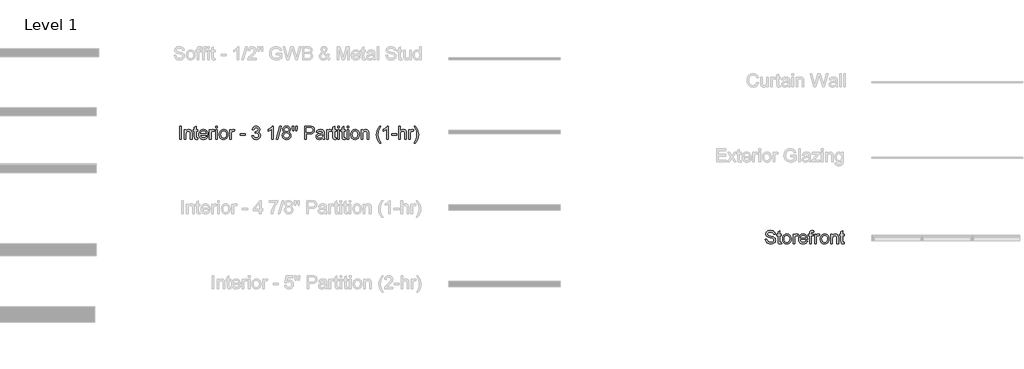
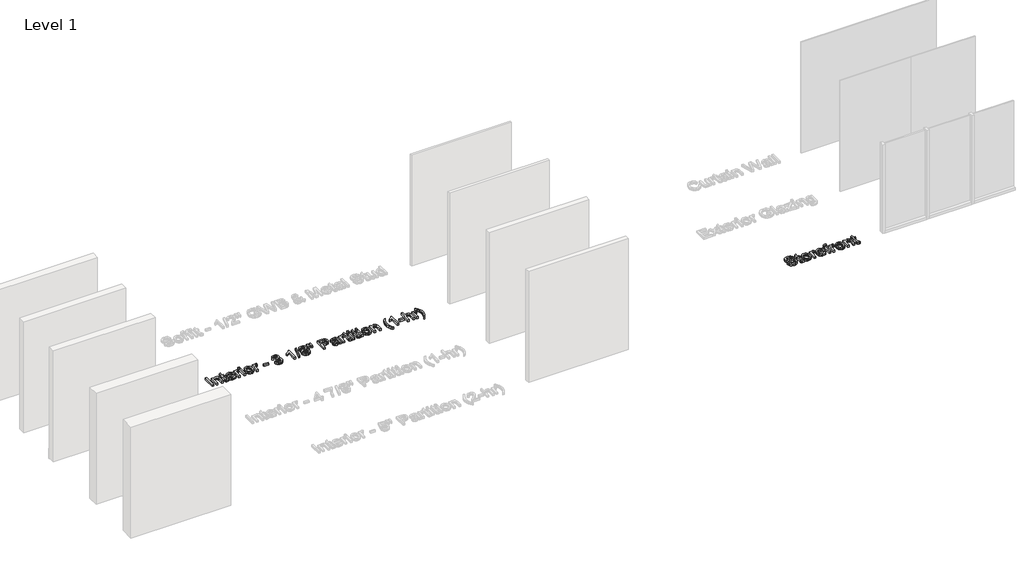
# One storey, part 36 of 42: 2 proxies.
"""IFC4 building model written with IfcOpenShell, lengths in millimetres."""

from ifc_helpers import new_model, si_unit, origin, origin_with_axes, place, context, project, spatial, polyline, outline, extrude, element, save

model = new_model("IFC4")

# Units and contexts
model_context = context("Model", 3, world=origin())
ifc_project = project(units=[si_unit("LENGTHUNIT", "METRE", prefix="MILLI")], contexts=[model_context])

# Site, building, storey
site = spatial("IfcSite", under=ifc_project)
building = spatial("IfcBuilding", under=site)
storey = spatial("IfcBuildingStorey", under=building, Name="Level 1", Elevation=0.0)

# Proxies
placement = place(None, origin())
element("IfcBuildingElementProxy", 1, Name="8\" Arial", ObjectType="8\" Arial", at=placement, inside=storey, context=model_context, shape_type="SweptSolid", body=[
    extrude(outline(polyline([(5241.2577476, 15464.2109771), (5241.2577476, 15768.7780711), (5279.3286344, 15768.7780711), (5279.3286344, 15464.2109771), (5241.2577476, 15464.2109771)])), origin_with_axes(), (0.0, 0.0, 1.0), 50.8),
    extrude(outline(polyline([(5350.711547, 15464.2109771), (5350.711547, 15687.8774368), (5388.7824338, 15687.8774368), (5388.7824338, 15656.6474125), (5402.0087209, 15672.3925497), (5417.8932779, 15683.6390763), (5436.4361048, 15690.3869923), (5457.6372016, 15692.6362976), (5476.4031002, 15690.8238408), (5493.5889082, 15685.3864705), (5507.9212586, 15677.0026962), (5518.1267844, 15666.3510272), (5529.5406147, 15638.3555411), (5531.5482591, 15601.5487268), (5531.5482591, 15464.2109771), (5493.4773724, 15464.2109771), (5493.4773724, 15596.4180799), (5489.0902975, 15630.1018918), (5483.020891, 15640.1308193), (5473.5868212, 15647.9104414), (5461.4944814, 15652.9016685), (5447.4502651, 15654.5654109), (5425.1523996, 15650.8289615), (5406.1448402, 15639.6196135), (5398.5487874, 15630.4690305), (5393.1230354, 15617.9630788), (5388.7824338, 15582.8850694), (5388.7824338, 15464.2109771), (5350.711547, 15464.2109771)])), origin_with_axes(), (0.0, 0.0, 1.0), 50.8),
    extrude(outline(polyline([(5664.7963628, 15495.9615018), (5669.5552236, 15463.0956191), (5641.0764158, 15459.4521162), (5622.8031337, 15461.0322067), (5609.1771767, 15465.7724783), (5599.5479192, 15473.0780732), (5593.2647357, 15482.354134), (5589.8071259, 15498.2851643), (5588.6545893, 15525.5556676), (5588.6545893, 15649.80655), (5560.1014242, 15649.80655), (5560.1014242, 15687.8774368), (5588.6545893, 15687.8774368), (5588.6545893, 15742.2325505), (5626.725476, 15764.6140679), (5626.725476, 15687.8774368), (5664.7963628, 15687.8774368), (5664.7963628, 15649.80655), (5626.725476, 15649.80655), (5626.725476, 15526.6710256), (5628.7331204, 15507.0407247), (5635.2393755, 15500.0883264), (5648.214707, 15497.523003), (5664.7963628, 15495.9615018)])), origin_with_axes(), (0.0, 0.0, 1.0), 50.8),
    extrude(outline(polyline([(5859.4635142, 15530.8350289), (5896.790829, 15526.076168), (5883.3414703, 15497.9505569), (5861.8801232, 15476.9260584), (5832.8901096, 15463.8206018), (5796.8547512, 15459.4521162), (5773.232398, 15461.3366065), (5752.1846629, 15466.9900774), (5733.7115459, 15476.412529), (5717.8130469, 15489.6039611), (5705.0282557, 15506.1972352), (5695.896262, 15525.8252125), (5690.4170658, 15548.4878931), (5688.590667, 15574.1852769), (5690.4356551, 15600.7540342), (5695.9706192, 15624.1719051), (5705.1955594, 15644.4388896), (5718.1104757, 15661.5549877), (5733.9671487, 15675.1530608), (5752.0173592, 15684.8659701), (5772.2611071, 15690.6937157), (5794.6983924, 15692.6362976), (5816.4130187, 15690.6983631), (5836.0502907, 15684.8845594), (5853.6102083, 15675.1948867), (5869.0927717, 15661.6293449), (5881.7311722, 15644.5504254), (5890.7586011, 15624.3206195), (5896.1750584, 15600.9399272), (5897.9805442, 15574.4083485), (5897.7574726, 15564.1470548), (5726.6615538, 15564.1470548), (5733.2514607, 15535.6496576), (5748.5597494, 15514.6995163), (5770.6531326, 15501.8171313), (5797.5983232, 15497.523003), (5817.8606604, 15499.5120581), (5834.925638, 15505.4792234), (5848.7932559, 15515.796285), (5859.4635142, 15530.8350289)]), holes=[polyline([(5726.6615538, 15602.2179416), (5859.9096574, 15602.2179416), (5854.7604213, 15622.3315644), (5844.6664313, 15636.7196827), (5822.4708069, 15650.1039788), (5794.549678, 15654.5654109), (5768.8871491, 15651.0055599), (5747.667463, 15640.3260069), (5732.9168533, 15623.6792886), (5726.6615538, 15602.2179416)])]), origin_with_axes(), (0.0, 0.0, 1.0), 50.8),
    extrude(outline(polyline([(5936.0514309, 15464.2109771), (5936.0514309, 15687.8774368), (5969.3634569, 15687.8774368), (5969.3634569, 15654.7884825), (5981.6695736, 15673.9726402), (5993.0090467, 15685.2749347), (6004.3856984, 15690.7959569), (6016.8033509, 15692.6362976), (6035.7644371, 15689.6991882), (6055.0229521, 15680.8878599), (6042.3078707, 15646.7579048), (6028.9235746, 15652.6135343), (6015.5392785, 15654.5654109), (6004.1719214, 15652.6878915), (5994.0128689, 15647.0553336), (5985.8056929, 15638.0952909), (5980.2939654, 15626.2353174), (5975.6652296, 15604.969158), (5974.1223177, 15581.7697114), (5974.1223177, 15464.2109771), (5936.0514309, 15464.2109771)])), origin_with_axes(), (0.0, 0.0, 1.0), 50.8),
    extrude(outline(polyline([(6078.8172563, 15730.7071844), (6078.8172563, 15768.7780711), (6116.888143, 15768.7780711), (6116.888143, 15730.7071844), (6078.8172563, 15730.7071844)])), origin_with_axes(), (0.0, 0.0, 1.0), 50.8),
    extrude(outline(polyline([(6078.8172563, 15464.2109771), (6078.8172563, 15687.8774368), (6116.888143, 15687.8774368), (6116.888143, 15464.2109771), (6078.8172563, 15464.2109771)])), origin_with_axes(), (0.0, 0.0, 1.0), 50.8),
    extrude(outline(polyline([(6164.4767515, 15576.0442069), (6166.5355165, 15605.0109839), (6172.7118115, 15629.9717667), (6183.0056364, 15650.9265553), (6197.4169914, 15667.8753498), (6211.9259402, 15678.7082645), (6227.9406223, 15686.4460607), (6245.4610377, 15691.0887384), (6264.4871864, 15692.6362976), (6285.490772, 15690.7518073), (6304.4820658, 15685.0983364), (6321.4610678, 15675.6758849), (6336.4277781, 15662.4844527), (6348.643272, 15645.9701832), (6357.3686248, 15626.5792194), (6362.6038364, 15604.3115615), (6364.348907, 15579.1672093), (6361.2630831, 15540.7059473), (6352.0056117, 15511.4277995), (6336.8460374, 15489.5017199), (6316.0539051, 15473.0966625), (6291.3580198, 15462.8632528), (6264.4871864, 15459.4521162), (6243.1768774, 15461.3296355), (6224.0089853, 15466.9621935), (6206.98351, 15476.3497901), (6192.1004516, 15489.4924253), (6180.0150828, 15506.1670276), (6171.3826765, 15526.1505252), (6166.2032327, 15549.4429184), (6164.4767515, 15576.0442069)]), holes=[polyline([(6202.5476383, 15576.1185641), (6206.9533024, 15541.6632962), (6220.1702948, 15517.1161254), (6240.060846, 15502.4212836), (6264.4871864, 15497.523003), (6288.8019911, 15502.4491675), (6308.6553637, 15517.2276612), (6321.8723561, 15542.1001448), (6326.2780202, 15577.3082793), (6321.8444721, 15610.759725), (6308.5438279, 15634.9722885), (6288.6625713, 15649.6671303), (6264.4871864, 15654.5654109), (6240.060846, 15649.6857196), (6220.1702948, 15635.0466457), (6206.9533024, 15610.5552427), (6202.5476383, 15576.1185641)])]), origin_with_axes(), (0.0, 0.0, 1.0), 50.8),
    extrude(outline(polyline([(6407.1786546, 15464.2109771), (6407.1786546, 15687.8774368), (6440.4906805, 15687.8774368), (6440.4906805, 15654.7884825), (6452.7967972, 15673.9726402), (6464.1362703, 15685.2749347), (6475.512922, 15690.7959569), (6487.9305745, 15692.6362976), (6506.8916607, 15689.6991882), (6526.1501757, 15680.8878599), (6513.4350944, 15646.7579048), (6500.0507983, 15652.6135343), (6486.6665021, 15654.5654109), (6475.2991451, 15652.6878915), (6465.1400925, 15647.0553336), (6456.9329165, 15638.0952909), (6451.421189, 15626.2353174), (6446.7924533, 15604.969158), (6445.2495413, 15581.7697114), (6445.2495413, 15464.2109771), (6407.1786546, 15464.2109771)])), origin_with_axes(), (0.0, 0.0, 1.0), 50.8),
    extrude(outline(polyline([(6649.8805577, 15554.6293331), (6649.8805577, 15592.7002199), (6768.8520788, 15592.7002199), (6768.8520788, 15554.6293331), (6649.8805577, 15554.6293331)])), origin_with_axes(), (0.0, 0.0, 1.0), 50.8),
    extrude(outline(polyline([(6921.1356258, 15545.1116114), (6959.2065126, 15549.8704723), (6967.7297067, 15525.9460429), (6980.2124218, 15509.7919411), (6997.2681047, 15500.5902375), (7019.5102023, 15497.523003), (7045.6095798, 15501.7427741), (7065.7603812, 15514.4020875), (7078.6427662, 15533.2888165), (7082.9368945, 15556.1908343), (7078.6799448, 15577.9310209), (7065.9090956, 15595.5629721), (7046.5762234, 15607.2463473), (7022.6332048, 15611.1408056), (6995.9389697, 15606.9768024), (7000.1773302, 15645.0476892), (7006.2746206, 15644.601546), (7029.0836919, 15647.3341731), (7049.4761542, 15655.5320545), (7063.8642726, 15669.3996724), (7068.660312, 15689.1415092), (7065.1841129, 15705.5837452), (7054.7555155, 15718.9215681), (7038.8430745, 15727.7607803), (7018.9153447, 15730.7071844), (6998.9504364, 15727.7328963), (6982.6290308, 15718.8100323), (6970.7132894, 15703.9385921), (6963.9653734, 15683.1185759), (6925.8944867, 15687.8774368), (6937.1038347, 15722.0631598), (6957.0501538, 15747.5862689), (6984.3392464, 15763.4801206), (7017.5769151, 15768.7780711), (7041.5106391, 15766.1662745), (7063.4924866, 15758.3308844), (7082.0260188, 15745.9689998), (7095.6147973, 15729.7777194), (7103.9520984, 15711.1233566), (7106.7311988, 15691.3722252), (7104.0915181, 15672.968818), (7096.1724763, 15656.2756265), (7083.0856089, 15642.0548118), (7064.942452, 15631.0685354), (7088.7739348, 15621.4392779), (7106.43377, 15605.0435152), (7117.3642785, 15582.7735336), (7121.0077813, 15555.5216195), (7119.1860299, 15536.2073366), (7113.7207756, 15518.4173764), (7104.6120185, 15502.1517387), (7091.8597586, 15487.4104237), (7076.323751, 15475.1786642), (7058.8637508, 15466.4416931), (7039.4797581, 15461.1995104), (7018.1717727, 15459.4521162), (6998.9132578, 15460.9439076), (6981.3649584, 15465.4192816), (6965.5268746, 15472.8782383), (6951.3990065, 15483.3207776), (6939.552975, 15496.1334528), (6930.560401, 15510.7028168), (6924.4212846, 15527.0288697), (6921.1356258, 15545.1116114)])), origin_with_axes(), (0.0, 0.0, 1.0), 50.8),
    extrude(outline(polyline([(7416.0571537, 15464.2109771), (7377.9862669, 15464.2109771), (7377.9862669, 15701.5591617), (7341.9230246, 15675.8687489), (7301.8444934, 15656.6474125), (7301.8444934, 15692.6362976), (7331.7453827, 15708.9019353), (7357.6495725, 15728.2533967), (7378.0699188, 15748.831752), (7391.5192774, 15768.7780711), (7416.0571537, 15768.7780711), (7416.0571537, 15464.2109771)])), origin_with_axes(), (0.0, 0.0, 1.0), 50.8),
    extrude(outline(polyline([(7487.4400664, 15464.2109771), (7573.0995616, 15768.7780711), (7607.4525883, 15768.7780711), (7521.7930931, 15464.2109771), (7487.4400664, 15464.2109771)])), origin_with_axes(), (0.0, 0.0, 1.0), 50.8),
    extrude(outline(polyline([(7680.9175026, 15631.9608218), (7660.5343349, 15641.9990439), (7646.2298684, 15655.6064117), (7637.7810315, 15672.5040855), (7634.9647525, 15692.413226), (7636.4983698, 15707.939939), (7641.0992216, 15722.1746956), (7648.7673079, 15735.1174958), (7659.5026288, 15746.7683397), (7672.7893311, 15756.3975972), (7688.1115617, 15763.2756383), (7724.8626082, 15768.7780711), (7761.8367262, 15763.1455132), (7777.3262606, 15756.1048157), (7790.8174452, 15746.2478393), (7801.7479537, 15734.3692765), (7809.5554598, 15721.2638199), (7814.2399634, 15706.9314694), (7815.8014646, 15691.3722252), (7813.0223643, 15672.1044156), (7804.6850631, 15655.4948759), (7790.6966148, 15641.97116), (7770.9640726, 15631.9608218), (7794.3958855, 15619.8870714), (7811.4515684, 15602.1064058), (7821.8522819, 15579.4739328), (7825.3191863, 15552.8447603), (7823.5996761, 15533.8557902), (7818.4411453, 15516.4469106), (7809.8435939, 15500.6181215), (7797.8070221, 15486.3694229), (7782.9634659, 15474.5931012), (7765.9449616, 15466.1814429), (7746.7515091, 15461.1344479), (7725.3831086, 15459.4521162), (7704.014708, 15461.1414189), (7684.8212556, 15466.2093268), (7667.8027513, 15474.6558401), (7652.9591951, 15486.4809587), (7640.9226232, 15500.8295747), (7632.3250719, 15516.8465805), (7627.1665411, 15534.531976), (7625.4470309, 15553.8857611), (7629.0533551, 15581.5466398), (7639.8723278, 15604.2999432), (7657.34627, 15621.3649207), (7680.9175026, 15631.9608218)]), holes=[polyline([(7663.5179176, 15555.2241907), (7665.1073028, 15540.659474), (7669.8754583, 15526.5594898), (7678.6774919, 15514.2626678), (7692.3685115, 15505.1074374), (7708.7642742, 15499.4191116), (7725.6805374, 15497.523003), (7751.5940218, 15501.5104079), (7771.0384298, 15513.4726225), (7783.1958321, 15531.5878955), (7787.2482996, 15554.0344755), (7783.065707, 15576.8621361), (7770.5179294, 15595.3770791), (7750.6273782, 15607.6460172), (7724.416465, 15611.7356633), (7698.8654719, 15607.7017851), (7679.6162516, 15595.6001507), (7667.5425011, 15577.4384044), (7663.5179176, 15555.2241907)]), polyline([(7673.0356393, 15691.297868), (7676.4095973, 15674.6790336), (7686.5314712, 15661.4062733), (7703.1038323, 15652.7064808), (7725.8292518, 15649.80655), (7748.0248762, 15652.6878915), (7764.3462818, 15661.3319161), (7774.3845039, 15674.1585332), (7777.7305779, 15689.5876524), (7774.2729681, 15705.6023345), (7763.9001386, 15718.8472109), (7747.3556614, 15727.742191), (7725.3831086, 15730.7071844), (7703.271136, 15727.8072535), (7686.7545428, 15719.1074611), (7676.4653652, 15706.3552011), (7673.0356393, 15691.297868)])]), origin_with_axes(), (0.0, 0.0, 1.0), 50.8),
    extrude(outline(polyline([(7867.9258623, 15659.3242717), (7858.6312122, 15718.1408175), (7858.6312122, 15768.7780711), (7896.702099, 15768.7780711), (7896.702099, 15718.1408175), (7888.3740925, 15659.3242717), (7867.9258623, 15659.3242717)])), origin_with_axes(), (0.0, 0.0, 1.0), 50.8),
    extrude(outline(polyline([(7943.8445643, 15659.3242717), (7934.7729858, 15718.1408175), (7934.7729858, 15768.7780711), (7972.8438725, 15768.7780711), (7972.8438725, 15718.1408175), (7963.9210084, 15659.3242717), (7943.8445643, 15659.3242717)])), origin_with_axes(), (0.0, 0.0, 1.0), 50.8),
    extrude(outline(polyline([(8144.1628629, 15464.2109771), (8144.1628629, 15768.7780711), (8257.0370936, 15768.7780711), (8302.5437004, 15765.8781403), (8322.8339216, 15760.4593593), (8339.5364078, 15751.6387364), (8352.9857665, 15739.0166015), (8363.516605, 15722.1932849), (8370.3202889, 15702.349207), (8372.5881835, 15680.6647883), (8371.0568899, 15661.9685996), (8366.4630091, 15644.7688497), (8358.8065411, 15629.0655383), (8348.0874859, 15614.8586657), (8333.3717311, 15603.082344), (8313.7251645, 15594.6706857), (8289.147786, 15589.6236907), (8259.6395956, 15587.941359), (8182.2337497, 15587.941359), (8182.2337497, 15464.2109771), (8144.1628629, 15464.2109771)]), holes=[polyline([(8182.2337497, 15626.0122458), (8261.8703116, 15626.0122458), (8295.6284808, 15629.5070342), (8317.935641, 15639.9913995), (8330.3718828, 15656.8147162), (8334.5172967, 15679.3263587), (8332.0728038, 15696.4285148), (8324.7393248, 15710.8538118), (8313.4277357, 15721.7099631), (8299.048912, 15728.1046823), (8260.9780252, 15730.7071844), (8182.2337497, 15730.7071844), (8182.2337497, 15626.0122458)])]), origin_with_axes(), (0.0, 0.0, 1.0), 50.8),
    extrude(outline(polyline([(8562.9426173, 15492.7641421), (8544.7529871, 15477.1677193), (8526.0242671, 15466.9621935), (8506.3289036, 15461.3296355), (8485.2393426, 15459.4521162), (8453.4237553, 15463.9693162), (8429.9547638, 15477.520916), (8415.4829936, 15498.0992713), (8410.6590702, 15523.6967376), (8412.4808217, 15539.4790535), (8417.9460759, 15553.8114039), (8426.3763235, 15566.080342), (8437.0930551, 15575.6724209), (8463.7501115, 15588.1644306), (8496.6903515, 15593.8899351), (8535.616346, 15599.9128683), (8562.7195457, 15606.9768024), (8562.9426173, 15615.4535233), (8560.321526, 15632.4441436), (8552.458252, 15643.5605451), (8534.872774, 15651.8141944), (8510.3720764, 15654.5654109), (8487.6931302, 15652.7343648), (8471.8550464, 15647.2412266), (8461.054663, 15637.082174), (8453.4888179, 15621.2533849), (8415.4179311, 15626.0122458), (8422.0264273, 15646.832262), (8431.888051, 15663.1908461), (8445.9229727, 15675.7014452), (8465.0513626, 15684.9775059), (8488.4459968, 15690.7215997), (8515.2796516, 15692.6362976), (8541.0165377, 15690.9446713), (8561.4182947, 15685.8697923), (8576.8009406, 15678.2388846), (8587.4804935, 15668.879172), (8594.5630169, 15657.3073326), (8599.154574, 15643.0400447), (8601.013504, 15609.7280188), (8601.013504, 15562.362482), (8602.9467913, 15496.221752), (8610.5312257, 15464.2109771), (8572.460339, 15464.2109771), (8566.3630485, 15477.4465588), (8562.9426173, 15492.7641421)]), holes=[polyline([(8562.9426173, 15568.9059156), (8501.5235695, 15557.2318351), (8468.7692226, 15551.0601875), (8453.9349611, 15541.0219654), (8448.729957, 15526.3735968), (8451.5648253, 15515.052713), (8460.0694301, 15505.7766523), (8474.0578785, 15499.5864153), (8493.3442774, 15497.523003), (8513.7925076, 15499.8001922), (8531.8613074, 15506.6317601), (8546.5096759, 15516.6978661), (8556.6966124, 15528.6786701), (8561.2138124, 15541.0219654), (8562.7195457, 15558.1241215), (8562.9426173, 15568.9059156)])]), origin_with_axes(), (0.0, 0.0, 1.0), 50.8),
    extrude(outline(polyline([(8653.3609733, 15464.2109771), (8653.3609733, 15687.8774368), (8686.6729992, 15687.8774368), (8686.6729992, 15654.7884825), (8698.979116, 15673.9726402), (8710.3185891, 15685.2749347), (8721.6952408, 15690.7959569), (8734.1128933, 15692.6362976), (8753.0739795, 15689.6991882), (8772.3324945, 15680.8878599), (8759.6174131, 15646.7579048), (8746.233117, 15652.6135343), (8732.8488209, 15654.5654109), (8721.4814638, 15652.6878915), (8711.3224113, 15647.0553336), (8703.1152353, 15638.0952909), (8697.6035078, 15626.2353174), (8692.974772, 15604.969158), (8691.4318601, 15581.7697114), (8691.4318601, 15464.2109771), (8653.3609733, 15464.2109771)])), origin_with_axes(), (0.0, 0.0, 1.0), 50.8),
    extrude(outline(polyline([(8877.027433, 15495.9615018), (8881.7862939, 15463.0956191), (8853.307486, 15459.4521162), (8835.0342039, 15461.0322067), (8821.4082469, 15465.7724783), (8811.7789894, 15473.0780732), (8805.495806, 15482.354134), (8802.0381961, 15498.2851643), (8800.8856595, 15525.5556676), (8800.8856595, 15649.80655), (8772.3324945, 15649.80655), (8772.3324945, 15687.8774368), (8800.8856595, 15687.8774368), (8800.8856595, 15742.2325505), (8838.9565463, 15764.6140679), (8838.9565463, 15687.8774368), (8877.027433, 15687.8774368), (8877.027433, 15649.80655), (8838.9565463, 15649.80655), (8838.9565463, 15526.6710256), (8840.9641907, 15507.0407247), (8847.4704458, 15500.0883264), (8860.4457773, 15497.523003), (8877.027433, 15495.9615018)])), origin_with_axes(), (0.0, 0.0, 1.0), 50.8),
    extrude(outline(polyline([(8915.0983198, 15730.7071844), (8915.0983198, 15768.7780711), (8953.1692066, 15768.7780711), (8953.1692066, 15730.7071844), (8915.0983198, 15730.7071844)])), origin_with_axes(), (0.0, 0.0, 1.0), 50.8),
    extrude(outline(polyline([(8915.0983198, 15464.2109771), (8915.0983198, 15687.8774368), (8953.1692066, 15687.8774368), (8953.1692066, 15464.2109771), (8915.0983198, 15464.2109771)])), origin_with_axes(), (0.0, 0.0, 1.0), 50.8),
    extrude(outline(polyline([(9091.1761711, 15495.9615018), (9095.9350319, 15463.0956191), (9067.456224, 15459.4521162), (9049.182942, 15461.0322067), (9035.5569849, 15465.7724783), (9025.9277274, 15473.0780732), (9019.644544, 15482.354134), (9016.1869342, 15498.2851643), (9015.0343975, 15525.5556676), (9015.0343975, 15649.80655), (8986.4812325, 15649.80655), (8986.4812325, 15687.8774368), (9015.0343975, 15687.8774368), (9015.0343975, 15742.2325505), (9053.1052843, 15764.6140679), (9053.1052843, 15687.8774368), (9091.1761711, 15687.8774368), (9091.1761711, 15649.80655), (9053.1052843, 15649.80655), (9053.1052843, 15526.6710256), (9055.1129287, 15507.0407247), (9061.6191838, 15500.0883264), (9074.5945153, 15497.523003), (9091.1761711, 15495.9615018)])), origin_with_axes(), (0.0, 0.0, 1.0), 50.8),
    extrude(outline(polyline([(9129.2470578, 15464.2109771), (9129.2470578, 15687.8774368), (9167.3179446, 15687.8774368), (9167.3179446, 15464.2109771), (9129.2470578, 15464.2109771)])), origin_with_axes(), (0.0, 0.0, 1.0), 50.8),
    extrude(outline(polyline([(9129.2470578, 15730.7071844), (9129.2470578, 15768.7780711), (9167.3179446, 15768.7780711), (9167.3179446, 15730.7071844), (9129.2470578, 15730.7071844)])), origin_with_axes(), (0.0, 0.0, 1.0), 50.8),
    extrude(outline(polyline([(9214.906553, 15576.0442069), (9216.965318, 15605.0109839), (9223.141613, 15629.9717667), (9233.435438, 15650.9265553), (9247.8467929, 15667.8753498), (9262.3557417, 15678.7082645), (9278.3704238, 15686.4460607), (9295.8908392, 15691.0887384), (9314.916988, 15692.6362976), (9335.9205735, 15690.7518073), (9354.9118673, 15685.0983364), (9371.8908693, 15675.6758849), (9386.8575796, 15662.4844527), (9399.0730735, 15645.9701832), (9407.7984263, 15626.5792194), (9413.033638, 15604.3115615), (9414.7787085, 15579.1672093), (9411.6928847, 15540.7059473), (9402.4354132, 15511.4277995), (9387.2758389, 15489.5017199), (9366.4837066, 15473.0966625), (9341.7878214, 15462.8632528), (9314.916988, 15459.4521162), (9293.606679, 15461.3296355), (9274.4387868, 15466.9621935), (9257.4133115, 15476.3497901), (9242.5302531, 15489.4924253), (9230.4448843, 15506.1670276), (9221.812478, 15526.1505252), (9216.6330343, 15549.4429184), (9214.906553, 15576.0442069)]), holes=[polyline([(9252.9774398, 15576.1185641), (9257.3831039, 15541.6632962), (9270.6000963, 15517.1161254), (9290.4906475, 15502.4212836), (9314.916988, 15497.523003), (9339.2317926, 15502.4491675), (9359.0851652, 15517.2276612), (9372.3021576, 15542.1001448), (9376.7078217, 15577.3082793), (9372.2742737, 15610.759725), (9358.9736294, 15634.9722885), (9339.0923728, 15649.6671303), (9314.916988, 15654.5654109), (9290.4906475, 15649.6857196), (9270.6000963, 15635.0466457), (9257.3831039, 15610.5552427), (9252.9774398, 15576.1185641)])]), origin_with_axes(), (0.0, 0.0, 1.0), 50.8),
    extrude(outline(polyline([(9457.6084561, 15464.2109771), (9457.6084561, 15687.8774368), (9495.6793429, 15687.8774368), (9495.6793429, 15656.6474125), (9508.9056299, 15672.3925497), (9524.7901869, 15683.6390763), (9543.3330139, 15690.3869923), (9564.5341107, 15692.6362976), (9583.3000092, 15690.8238408), (9600.4858173, 15685.3864705), (9614.8181677, 15677.0026962), (9625.0236935, 15666.3510272), (9636.4375238, 15638.3555411), (9638.4451682, 15601.5487268), (9638.4451682, 15464.2109771), (9600.3742815, 15464.2109771), (9600.3742815, 15596.4180799), (9595.9872066, 15630.1018918), (9589.9178001, 15640.1308193), (9580.4837303, 15647.9104414), (9568.3913905, 15652.9016685), (9554.3471742, 15654.5654109), (9532.0493087, 15650.8289615), (9513.0417492, 15639.6196135), (9505.4456964, 15630.4690305), (9500.0199445, 15617.9630788), (9495.6793429, 15582.8850694), (9495.6793429, 15464.2109771), (9457.6084561, 15464.2109771)])), origin_with_axes(), (0.0, 0.0, 1.0), 50.8),
    extrude(outline(polyline([(9885.9059321, 15378.5514819), (9856.4047128, 15419.9498533), (9831.8482472, 15467.8544799), (9815.2851808, 15519.941699), (9809.7641586, 15573.8878481), (9813.8909833, 15621.197617), (9826.2714572, 15666.462563), (9850.846512, 15717.7318528), (9885.9059321, 15768.7780711), (9914.4590972, 15768.7780711), (9878.8419981, 15708.4743814), (9857.4271243, 15650.0296216), (9850.2330651, 15611.9401456), (9847.8350454, 15573.6647765), (9851.9990486, 15524.8585689), (9864.4910583, 15476.0709506), (9885.3110745, 15427.3019216), (9914.4590972, 15378.5514819), (9885.9059321, 15378.5514819)])), origin_with_axes(), (0.0, 0.0, 1.0), 50.8),
    extrude(outline(polyline([(10085.7780876, 15464.2109771), (10047.7072009, 15464.2109771), (10047.7072009, 15701.5591617), (10011.6439585, 15675.8687489), (9971.5654273, 15656.6474125), (9971.5654273, 15692.6362976), (10001.4663167, 15708.9019353), (10027.3705065, 15728.2533967), (10047.7908527, 15748.831752), (10061.2402114, 15768.7780711), (10085.7780876, 15768.7780711), (10085.7780876, 15464.2109771)])), origin_with_axes(), (0.0, 0.0, 1.0), 50.8),
    extrude(outline(polyline([(10166.678722, 15554.6293331), (10166.678722, 15592.7002199), (10285.6502431, 15592.7002199), (10285.6502431, 15554.6293331), (10166.678722, 15554.6293331)])), origin_with_axes(), (0.0, 0.0, 1.0), 50.8),
    extrude(outline(polyline([(10328.4799907, 15464.2109771), (10328.4799907, 15768.7780711), (10366.5508775, 15768.7780711), (10366.5508775, 15656.7961269), (10380.5346785, 15672.4762016), (10396.2379898, 15683.6762549), (10413.6608114, 15690.3962869), (10432.8031433, 15692.6362976), (10455.7981076, 15690.1918046), (10475.5585337, 15682.8583257), (10491.1177779, 15671.2121292), (10501.5091967, 15655.8294833), (10507.3648263, 15634.693449), (10509.3167028, 15605.7870872), (10509.3167028, 15464.2109771), (10471.2458161, 15464.2109771), (10471.2458161, 15601.8461556), (10468.2157601, 15625.6776384), (10459.1255923, 15641.9990439), (10444.4772238, 15651.4238191), (10424.7725656, 15654.5654109), (10408.6835263, 15652.4462306), (10393.5797199, 15646.08869), (10381.0691209, 15636.1062358), (10372.7597037, 15623.112315), (10368.103084, 15605.8428551), (10366.5508775, 15583.0337838), (10366.5508775, 15464.2109771), (10328.4799907, 15464.2109771)])), origin_with_axes(), (0.0, 0.0, 1.0), 50.8),
    extrude(outline(polyline([(10561.6641721, 15464.2109771), (10561.6641721, 15687.8774368), (10594.976198, 15687.8774368), (10594.976198, 15654.7884825), (10607.2823147, 15673.9726402), (10618.6217878, 15685.2749347), (10629.9984395, 15690.7959569), (10642.4160921, 15692.6362976), (10661.3771782, 15689.6991882), (10680.6356932, 15680.8878599), (10667.9206119, 15646.7579048), (10654.5363158, 15652.6135343), (10641.1520197, 15654.5654109), (10629.7846626, 15652.6878915), (10619.6256101, 15647.0553336), (10611.418434, 15638.0952909), (10605.9067065, 15626.2353174), (10601.2779708, 15604.969158), (10599.7350589, 15581.7697114), (10599.7350589, 15464.2109771), (10561.6641721, 15464.2109771)])), origin_with_axes(), (0.0, 0.0, 1.0), 50.8),
    extrude(outline(polyline([(10713.9477191, 15378.5514819), (10685.3945541, 15378.5514819), (10714.5425767, 15427.3019216), (10735.3625929, 15476.0709506), (10747.8546027, 15524.8585689), (10752.0186059, 15573.6647765), (10749.6205862, 15611.661306), (10742.426527, 15649.3604068), (10733.3363592, 15679.2334122), (10721.2347248, 15707.8795238), (10685.3945541, 15768.7780711), (10713.9477191, 15768.7780711), (10749.0071393, 15717.7318528), (10773.5821941, 15666.462563), (10785.962668, 15621.197617), (10790.0894927, 15573.8878481), (10784.5405866, 15519.941699), (10767.8938682, 15467.8544799), (10743.3095188, 15419.9498533), (10713.9477191, 15378.5514819)])), origin_with_axes(), (0.0, 0.0, 1.0), 50.8),
])
element("IfcBuildingElementProxy", 2, Name="8\" Arial", ObjectType="8\" Arial", at=placement, inside=storey, context=model_context, shape_type="SweptSolid", body=[
    extrude(outline(polyline([(18840.5112863, 13143.7956167), (18878.582173, 13143.7956167), (18882.9506586, 13122.6688771), (18890.8511111, 13105.6875513), (18903.1758171, 13092.2103087), (18920.817063, 13081.5958183), (18942.3806512, 13074.7084826), (18966.4723842, 13072.412704), (18987.6827757, 13074.1508036), (19006.2534866, 13079.3651023), (19021.3015251, 13087.6187516), (19031.9438995, 13098.4749029), (19038.2735562, 13110.9390286), (19040.3834417, 13124.0166013), (19038.8033512, 13136.7595666), (19034.0630797, 13147.7737269), (19024.4338222, 13157.1706182), (19008.1867738, 13165.0617761), (18952.7534807, 13179.5986088), (18916.3649256, 13189.2185717), (18893.0818271, 13198.373802), (18874.1300356, 13211.1818298), (18860.6992662, 13226.7038955), (18852.6965725, 13244.6053916), (18850.0290079, 13264.5517106), (18853.3286087, 13286.8495762), (18863.2274111, 13307.6417085), (18879.4651648, 13325.264365), (18901.7816196, 13338.0538035), (18928.5688012, 13345.8334257), (18958.218735, 13348.426633), (18990.3410457, 13345.7125952), (19018.4480675, 13337.5704817), (19041.5359783, 13324.1675963), (19058.6009559, 13305.6712426), (19069.4013393, 13283.2339573), (19073.6954676, 13258.008277), (19035.6245809, 13258.008277), (19028.635004, 13280.7244018), (19014.0609927, 13297.1201646), (18991.2891, 13307.0468508), (18959.705879, 13310.3557463), (18927.379086, 13307.0840294), (18905.2020509, 13297.268879), (18892.3754337, 13282.8249927), (18888.0998947, 13265.6670687), (18891.1299506, 13251.0372894), (18900.2201184, 13239.2702624), (18921.7093494, 13228.7487185), (18962.3827382, 13218.004103), (19004.357378, 13207.7985772), (19029.750362, 13198.8943024), (19051.45337, 13185.0824524), (19066.594355, 13168.0360641), (19075.4893351, 13147.9410306), (19078.4543285, 13124.9832449), (19075.0431919, 13101.5142535), (19064.8097822, 13079.4394595), (19048.1723585, 13060.4411947), (19025.5491802, 13046.2017908), (18998.3437394, 13037.3068107), (18967.9595283, 13034.3418173), (18930.6600975, 13037.5391769), (18899.9598682, 13047.1312558), (18875.5056438, 13063.1552325), (18856.9442276, 13085.6482858), (18845.0284862, 13113.0489142), (18840.5112863, 13143.7956167)])), origin_with_axes(), (0.0, 0.0, 1.0), 50.8),
    extrude(outline(polyline([(19211.7024321, 13070.8512028), (19216.461293, 13037.9853201), (19187.9824851, 13034.3418173), (19169.7092031, 13035.9219078), (19156.083246, 13040.6621793), (19146.4539885, 13047.9677743), (19140.1708051, 13057.2438351), (19136.7131952, 13073.1748653), (19135.5606586, 13100.4453687), (19135.5606586, 13224.6962511), (19107.0074936, 13224.6962511), (19107.0074936, 13262.7671378), (19135.5606586, 13262.7671378), (19135.5606586, 13317.1222515), (19173.6315454, 13339.503769), (19173.6315454, 13262.7671378), (19211.7024321, 13262.7671378), (19211.7024321, 13224.6962511), (19173.6315454, 13224.6962511), (19173.6315454, 13101.5607267), (19175.6391898, 13081.9304257), (19182.1454449, 13074.9780275), (19195.1207764, 13072.412704), (19211.7024321, 13070.8512028)])), origin_with_axes(), (0.0, 0.0, 1.0), 50.8),
    extrude(outline(polyline([(19240.2555972, 13150.933908), (19242.3143622, 13179.900685), (19248.4906572, 13204.8614678), (19258.7844822, 13225.8162564), (19273.1958371, 13242.7650508), (19287.7047859, 13253.5979655), (19303.719468, 13261.3357617), (19321.2398834, 13265.9784394), (19340.2660322, 13267.5259987), (19361.2696177, 13265.6415084), (19380.2609115, 13259.9880375), (19397.2399135, 13250.5655859), (19412.2066238, 13237.3741538), (19424.4221177, 13220.8598842), (19433.1474705, 13201.4689205), (19438.3826821, 13179.2012626), (19440.1277527, 13154.0569104), (19437.0419289, 13115.5956483), (19427.7844574, 13086.3175006), (19412.6248831, 13064.391421), (19391.8327508, 13047.9863636), (19367.1368656, 13037.7529539), (19340.2660322, 13034.3418173), (19318.9557232, 13036.2193366), (19299.787831, 13041.8518945), (19282.7623557, 13051.2394911), (19267.8792973, 13064.3821264), (19255.7939285, 13081.0567286), (19247.1615222, 13101.0402263), (19241.9820785, 13124.3326194), (19240.2555972, 13150.933908)]), holes=[polyline([(19278.326484, 13151.0082652), (19282.7321481, 13116.5529973), (19295.9491405, 13092.0058264), (19315.8396917, 13077.3109846), (19340.2660322, 13072.412704), (19364.5808368, 13077.3388686), (19384.4342094, 13092.1173622), (19397.6512018, 13116.9898459), (19402.0568659, 13152.1979804), (19397.6233178, 13185.6494261), (19384.3226736, 13209.8619895), (19364.441417, 13224.5568313), (19340.2660322, 13229.4551119), (19315.8396917, 13224.5754206), (19295.9491405, 13209.9363467), (19282.7321481, 13185.4449438), (19278.326484, 13151.0082652)])]), origin_with_axes(), (0.0, 0.0, 1.0), 50.8),
    extrude(outline(polyline([(19482.9575003, 13039.1006781), (19482.9575003, 13262.7671378), (19516.2695262, 13262.7671378), (19516.2695262, 13229.6781835), (19528.5756429, 13248.8623413), (19539.915116, 13260.1646358), (19551.2917677, 13265.685658), (19563.7094203, 13267.5259987), (19582.6705064, 13264.5888892), (19601.9290214, 13255.777561), (19589.2139401, 13221.6476058), (19575.829644, 13227.5032354), (19562.4453479, 13229.4551119), (19551.0779908, 13227.5775926), (19540.9189382, 13221.9450346), (19532.7117622, 13212.984992), (19527.2000347, 13201.1250184), (19522.571299, 13179.858859), (19521.0283871, 13156.6594124), (19521.0283871, 13039.1006781), (19482.9575003, 13039.1006781)])), origin_with_axes(), (0.0, 0.0, 1.0), 50.8),
    extrude(outline(polyline([(19782.3195903, 13105.7247299), (19819.6469051, 13100.9658691), (19806.1975464, 13072.8402579), (19784.7361993, 13051.8157594), (19755.7461857, 13038.7103028), (19719.7108273, 13034.3418173), (19696.0884741, 13036.2263076), (19675.040739, 13041.8797785), (19656.567622, 13051.30223), (19640.669123, 13064.4936622), (19627.8843318, 13081.0869362), (19618.7523381, 13100.7149136), (19613.2731419, 13123.3775941), (19611.4467431, 13149.074978), (19613.2917312, 13175.6437352), (19618.8266953, 13199.0616061), (19628.0516355, 13219.3285906), (19640.9665518, 13236.4446888), (19656.8232248, 13250.0427619), (19674.8734353, 13259.7556712), (19695.1171832, 13265.5834168), (19717.5544685, 13267.5259987), (19739.2690948, 13265.5880641), (19758.9063668, 13259.7742605), (19776.4662844, 13250.0845878), (19791.9488478, 13236.519046), (19804.5872483, 13219.4401264), (19813.6146772, 13199.2103205), (19819.0311345, 13175.8296282), (19820.8366203, 13149.2980496), (19820.6135487, 13139.0367559), (19649.5176299, 13139.0367559), (19656.1075368, 13110.5393587), (19671.4158255, 13089.5892174), (19693.5092087, 13076.7068324), (19720.4543993, 13072.412704), (19740.7167365, 13074.4017592), (19757.7817141, 13080.3689245), (19771.649332, 13090.6859861), (19782.3195903, 13105.7247299)]), holes=[polyline([(19649.5176299, 13177.1076426), (19782.7657335, 13177.1076426), (19777.6164974, 13197.2212654), (19767.5225074, 13211.6093837), (19745.326883, 13224.9936799), (19717.4057541, 13229.4551119), (19691.7432252, 13225.8952609), (19670.5235391, 13215.215708), (19655.7729294, 13198.5689897), (19649.5176299, 13177.1076426)])]), origin_with_axes(), (0.0, 0.0, 1.0), 50.8),
    extrude(outline(polyline([(19868.4252287, 13039.1006781), (19868.4252287, 13224.6962511), (19835.1132028, 13224.6962511), (19835.1132028, 13262.7671378), (19868.4252287, 13262.7671378), (19868.4252287, 13285.2973696), (19872.4405176, 13317.0478943), (19880.0993092, 13329.7072078), (19891.9221042, 13339.7268406), (19908.4665813, 13346.2516849), (19930.2904197, 13348.426633), (19965.0152324, 13344.2626298), (19959.4384424, 13308.5711735), (19937.5030682, 13310.3557463), (19923.031298, 13308.7756558), (19913.522871, 13304.0353842), (19908.2528044, 13294.982395), (19906.4961155, 13280.4641516), (19906.4961155, 13262.7671378), (19949.3258631, 13262.7671378), (19949.3258631, 13224.6962511), (19906.4961155, 13224.6962511), (19906.4961155, 13039.1006781), (19868.4252287, 13039.1006781)])), origin_with_axes(), (0.0, 0.0, 1.0), 50.8),
    extrude(outline(polyline([(19982.637889, 13039.1006781), (19982.637889, 13262.7671378), (20015.9499149, 13262.7671378), (20015.9499149, 13229.6781835), (20028.2560316, 13248.8623413), (20039.5955047, 13260.1646358), (20050.9721565, 13265.685658), (20063.389809, 13267.5259987), (20082.3508951, 13264.5888892), (20101.6094101, 13255.777561), (20088.8943288, 13221.6476058), (20075.5100327, 13227.5032354), (20062.1257366, 13229.4551119), (20050.7583795, 13227.5775926), (20040.599327, 13221.9450346), (20032.3921509, 13212.984992), (20026.8804234, 13201.1250184), (20022.2516877, 13179.858859), (20020.7087758, 13156.6594124), (20020.7087758, 13039.1006781), (19982.637889, 13039.1006781)])), origin_with_axes(), (0.0, 0.0, 1.0), 50.8),
    extrude(outline(polyline([(20115.8859927, 13150.933908), (20117.9447577, 13179.900685), (20124.1210526, 13204.8614678), (20134.4148776, 13225.8162564), (20148.8262326, 13242.7650508), (20163.3351814, 13253.5979655), (20179.3498635, 13261.3357617), (20196.8702789, 13265.9784394), (20215.8964276, 13267.5259987), (20236.9000131, 13265.6415084), (20255.8913069, 13259.9880375), (20272.870309, 13250.5655859), (20287.8370193, 13237.3741538), (20300.0525132, 13220.8598842), (20308.7778659, 13201.4689205), (20314.0130776, 13179.2012626), (20315.7581481, 13154.0569104), (20312.6723243, 13115.5956483), (20303.4148528, 13086.3175006), (20288.2552785, 13064.391421), (20267.4631463, 13047.9863636), (20242.767261, 13037.7529539), (20215.8964276, 13034.3418173), (20194.5861186, 13036.2193366), (20175.4182265, 13041.8518945), (20158.3927512, 13051.2394911), (20143.5096927, 13064.3821264), (20131.4243239, 13081.0567286), (20122.7919177, 13101.0402263), (20117.6124739, 13124.3326194), (20115.8859927, 13150.933908)]), holes=[polyline([(20153.9568794, 13151.0082652), (20158.3625436, 13116.5529973), (20171.579536, 13092.0058264), (20191.4700872, 13077.3109846), (20215.8964276, 13072.412704), (20240.2112322, 13077.3388686), (20260.0646048, 13092.1173622), (20273.2815972, 13116.9898459), (20277.6872614, 13152.1979804), (20273.2537133, 13185.6494261), (20259.953069, 13209.8619895), (20240.0718125, 13224.5568313), (20215.8964276, 13229.4551119), (20191.4700872, 13224.5754206), (20171.579536, 13209.9363467), (20158.3625436, 13185.4449438), (20153.9568794, 13151.0082652)])]), origin_with_axes(), (0.0, 0.0, 1.0), 50.8),
    extrude(outline(polyline([(20358.5878957, 13039.1006781), (20358.5878957, 13262.7671378), (20396.6587825, 13262.7671378), (20396.6587825, 13231.5371135), (20409.8850696, 13247.2822508), (20425.7696266, 13258.5287774), (20444.3124535, 13265.2766934), (20465.5135504, 13267.5259987), (20484.2794489, 13265.7135419), (20501.4652569, 13260.2761716), (20515.7976073, 13251.8923972), (20526.0031331, 13241.2407282), (20537.4169634, 13213.2452422), (20539.4246079, 13176.4384278), (20539.4246079, 13039.1006781), (20501.3537211, 13039.1006781), (20501.3537211, 13171.307781), (20496.9666463, 13204.9915929), (20490.8972397, 13215.0205203), (20481.4631699, 13222.8001425), (20469.3708301, 13227.7913695), (20455.3266139, 13229.4551119), (20433.0287483, 13225.7186626), (20414.0211889, 13214.5093146), (20406.4251361, 13205.3587316), (20400.9993841, 13192.8527799), (20396.6587825, 13157.7747704), (20396.6587825, 13039.1006781), (20358.5878957, 13039.1006781)])), origin_with_axes(), (0.0, 0.0, 1.0), 50.8),
    extrude(outline(polyline([(20672.6727115, 13070.8512028), (20677.4315724, 13037.9853201), (20648.9527645, 13034.3418173), (20630.6794824, 13035.9219078), (20617.0535254, 13040.6621793), (20607.4242679, 13047.9677743), (20601.1410844, 13057.2438351), (20597.6834746, 13073.1748653), (20596.530938, 13100.4453687), (20596.530938, 13224.6962511), (20567.9777729, 13224.6962511), (20567.9777729, 13262.7671378), (20596.530938, 13262.7671378), (20596.530938, 13317.1222515), (20634.6018247, 13339.503769), (20634.6018247, 13262.7671378), (20672.6727115, 13262.7671378), (20672.6727115, 13224.6962511), (20634.6018247, 13224.6962511), (20634.6018247, 13101.5607267), (20636.6094692, 13081.9304257), (20643.1157242, 13074.9780275), (20656.0910557, 13072.412704), (20672.6727115, 13070.8512028)])), origin_with_axes(), (0.0, 0.0, 1.0), 50.8),
])

save(model, "model.ifc")

# Revit data of these elements
# Elements 1, 2 (IfcBuildingElementProxy, "8\" Arial")
#   Phase Created = New Construction
